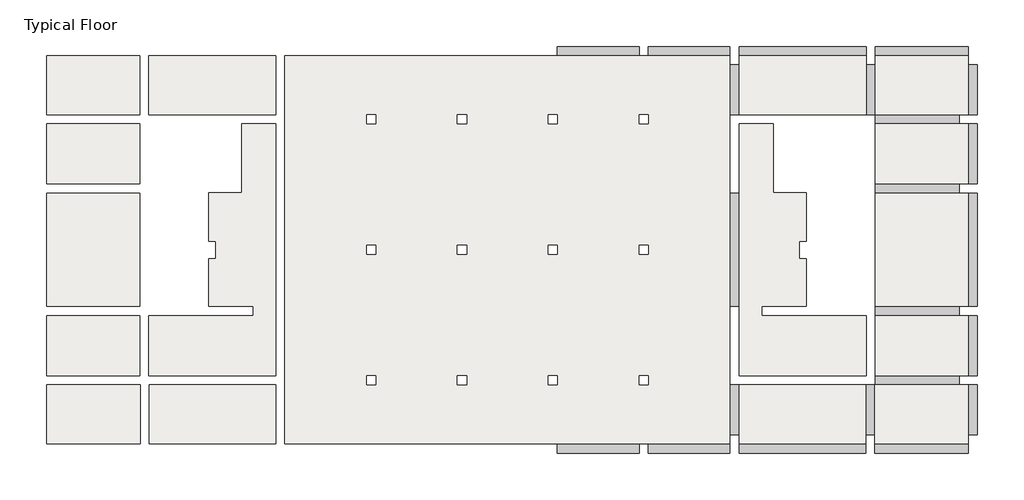
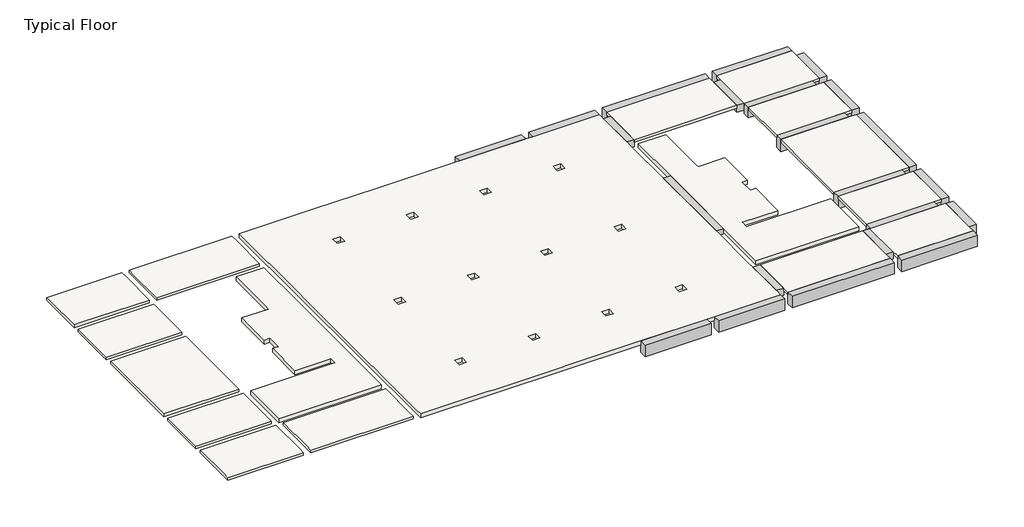
# One storey: 22 beams, 17 slabs.
"""IFC4 building model written with IfcOpenShell, lengths in millimetres."""

from ifc_helpers import new_model, si_unit, frame, origin, place, context, project, spatial, polyline, outline, extrude, faceted_brep, element, save

model = new_model("IFC4")

# Units and contexts
model_context = context("Model", 3, world=origin())
ifc_project = project(units=[si_unit("LENGTHUNIT", "METRE", prefix="MILLI")], contexts=[model_context])

# Site, building, storey
site = spatial("IfcSite", under=ifc_project)
building = spatial("IfcBuilding", under=site)
storey = spatial("IfcBuildingStorey", under=building, Name="Typical Floor", Elevation=4000.0)

# Beams
placement = place(None, origin())
element("IfcBeam", 1, ObjectType="Concrete Rectengular Beam : 40/30", at=placement, inside=storey, context=model_context, shape_type="SweptSolid", body=[
    extrude(outline(polyline([(9934.1113614, 5392.831899), (10334.1113614, 5392.831899), (10334.1113614, 443.9061014), (9934.1113614, 443.9061014), (9934.1113614, 5392.831899)])), frame((0.0, 0.0, 3700.0), z_axis=(0.0, 0.0, 1.0), x_axis=(1.0, 0.0, 0.0)), (0.0, 0.0, 1.0), 300.0),
])
element("IfcBeam", 2, ObjectType="Concrete Rectengular Beam : 40/40", at=placement, inside=storey, context=model_context, shape_type="Brep", body=[
    faceted_brep([(15855.0311968, -5152.7195656, 4000.0), (16255.0311968, -5152.7195656, 4000.0), (16255.0311968, -2974.5007845, 4000.0), (15855.0311968, -2974.5007845, 4000.0), (15855.0311968, -5152.7195656, 3600.0), (15855.0311968, -2974.5007845, 3600.0), (16255.0311968, -5152.7195656, 3600.0), (16255.0311968, -2974.5007845, 3600.0), (16255.0311968, -2974.5007845, 3850.0)], [[[0, 1, 2, 3]], [[4, 0, 3, 5]], [[6, 4, 5, 7]], [[1, 6, 7, 8, 2]], [[1, 0, 4, 6]], [[3, 2, 8, 7, 5]]]),
])
element("IfcBeam", 3, ObjectType="Concrete Rectengular Beam : 40/40", at=placement, inside=storey, context=model_context, shape_type="Brep", body=[
    faceted_brep([(9934.1113614, -5152.7195656, 4000.0), (10334.1113614, -5152.7195656, 4000.0), (10334.1113614, -2970.6647062, 4000.0), (9934.1113614, -2970.6647062, 4000.0), (9934.1113614, -5152.7195656, 3600.0), (9934.1113614, -2970.6647062, 3600.0), (10334.1113614, -5152.7195656, 3600.0), (10334.1113614, -2970.6647062, 3600.0), (10334.1113614, -2970.6647062, 3850.0)], [[[0, 1, 2, 3]], [[4, 0, 3, 5]], [[6, 4, 5, 7]], [[1, 6, 7, 8, 2]], [[1, 0, 4, 6]], [[3, 2, 8, 7, 5]]]),
])
element("IfcBeam", 4, ObjectType="Concrete Rectengular Beam : 40/40", at=placement, inside=storey, context=model_context, shape_type="Brep", body=[
    faceted_brep([(16276.5966375, 10981.7889465, 4000.0), (15876.5966375, 10981.7889465, 4000.0), (15876.5966375, 8813.6899891, 4000.0), (16276.5966375, 8813.6899891, 4000.0), (16276.5966375, 10981.7889465, 3600.0), (16276.5966375, 8813.6899891, 3850.0), (16276.5966375, 8813.6899891, 3600.0), (15876.5966375, 10981.7889465, 3600.0), (15876.5966375, 8813.6899891, 3600.0), (15876.5966375, 8813.6899891, 3850.0)], [[[0, 1, 2, 3]], [[4, 0, 3, 5, 6]], [[7, 4, 6, 8]], [[1, 7, 8, 9, 2]], [[1, 0, 4, 7]], [[3, 2, 9, 8, 6, 5]]]),
])
element("IfcBeam", 5, ObjectType="Concrete Rectengular Beam : 40/40", at=placement, inside=storey, context=model_context, shape_type="Brep", body=[
    faceted_brep([(10334.1113614, 10981.7889465, 4000.0), (9934.1113614, 10981.7889465, 4000.0), (9934.1113614, 8813.6899891, 4000.0), (10334.1113614, 8813.6899891, 4000.0), (10334.1113614, 10981.7889465, 3600.0), (10334.1113614, 8813.6899891, 3850.0), (10334.1113614, 8813.6899891, 3600.0), (9934.1113614, 10981.7889465, 3600.0), (9934.1113614, 8813.6899891, 3600.0)], [[[0, 1, 2, 3]], [[4, 0, 3, 5, 6]], [[7, 4, 6, 8]], [[1, 7, 8, 2]], [[1, 0, 4, 7]], [[3, 2, 8, 6, 5]]]),
])
element("IfcBeam", 6, ObjectType="Concrete Rectengular Beam : 40/60", at=placement, inside=storey, context=model_context, shape_type="Brep", body=[
    faceted_brep([(19935.0311968, 8413.6899891, 4000.0), (19935.0311968, 8813.6899891, 4000.0), (16276.5966375, 8813.6899891, 4000.0), (16276.5966375, 8413.6899891, 4000.0), (19935.0311968, 8413.6899891, 3400.0), (16276.5966375, 8413.6899891, 3850.0), (16276.5966375, 8413.6899891, 3400.0), (19935.0311968, 8813.6899891, 3400.0), (16276.5966375, 8813.6899891, 3400.0), (16276.5966375, 8813.6899891, 3850.0)], [[[0, 1, 2, 3]], [[4, 0, 3, 5, 6]], [[7, 4, 6, 8]], [[1, 7, 8, 9, 2]], [[1, 0, 4, 7]], [[3, 2, 9, 8, 6, 5]]]),
])
element("IfcBeam", 7, ObjectType="Concrete Rectengular Beam : 40/60", at=placement, inside=storey, context=model_context, shape_type="Brep", body=[
    faceted_brep([(19935.0311968, -2974.5007845, 4000.0), (19935.0311968, -2574.5007845, 4000.0), (16276.5966375, -2574.5007845, 4000.0), (16276.5966375, -2970.6647062, 4000.0), (15876.5966375, -2970.6647062, 4000.0), (15855.0311968, -2970.6647062, 4000.0), (15855.0311968, -2974.5007845, 4000.0), (16255.0311968, -2974.5007845, 4000.0), (19935.0311968, -2974.5007845, 3400.0), (15855.0311968, -2974.5007845, 3600.0), (15855.0311968, -2974.5007845, 3400.0), (19935.0311968, -2574.5007845, 3400.0), (15855.0311968, -2970.6647062, 3400.0), (16276.5966375, -2970.6647062, 3400.0), (16276.5966375, -2574.5007845, 3400.0), (15855.0311968, -2970.6647062, 3850.0), (16276.5966375, -2574.5007845, 3850.0)], [[[0, 1, 2, 3, 4, 5, 6, 7]], [[8, 0, 7, 6, 9, 10]], [[11, 8, 10, 12, 13, 14]], [[1, 0, 8, 11]], [[10, 9, 6, 5, 15, 12]], [[13, 3, 2, 16, 14]], [[3, 13, 12, 15, 5, 4]], [[1, 11, 14, 16, 2]]]),
])
element("IfcBeam", 8, ObjectType="Concrete Rectengular Beam : 40/65", at=placement, inside=storey, context=model_context, shape_type="Brep", body=[
    faceted_brep([(20335.0311968, 11381.7889465, 4000.0), (20335.0311968, 11781.7889465, 4000.0), (16276.5966375, 11781.7889465, 4000.0), (16276.5966375, 11381.7889465, 4000.0), (20335.0311968, 11781.7889465, 3350.0), (16276.5966375, 11781.7889465, 3350.0), (20335.0311968, 11381.7889465, 3350.0), (16276.5966375, 11381.7889465, 3350.0), (20335.0311968, 11381.7889465, 3850.0), (16276.5966375, 11381.7889465, 3850.0)], [[[0, 1, 2, 3]], [[1, 4, 5, 2]], [[4, 6, 7, 5]], [[6, 8, 0, 3, 9, 7]], [[1, 0, 8, 6, 4]], [[3, 2, 5, 7, 9]]]),
])
element("IfcBeam", 9, ObjectType="Concrete Rectengular Beam : 40/65", at=placement, inside=storey, context=model_context, shape_type="Brep", body=[
    faceted_brep([(15876.5966375, 11381.7889465, 4000.0), (15876.5966375, 11781.7889465, 4000.0), (10334.1113614, 11781.7889465, 4000.0), (10334.1113614, 11381.7889465, 4000.0), (15876.5966375, 11381.7889465, 3350.0), (15876.5966375, 11381.7889465, 3850.0), (10334.1113614, 11381.7889465, 3850.0), (10334.1113614, 11381.7889465, 3350.0), (15876.5966375, 11781.7889465, 3350.0), (10334.1113614, 11781.7889465, 3350.0)], [[[0, 1, 2, 3]], [[4, 5, 0, 3, 6, 7]], [[8, 4, 7, 9]], [[1, 8, 9, 2]], [[1, 0, 5, 4, 8]], [[3, 2, 9, 7, 6]]]),
])
element("IfcBeam", 10, ObjectType="Concrete Rectengular Beam : 40/65", at=placement, inside=storey, context=model_context, shape_type="Brep", body=[
    faceted_brep([(20335.0311968, -5948.8870638, 4000.0), (20335.0311968, -5548.8870638, 4000.0), (16255.0311968, -5548.8870638, 4000.0), (16255.0311968, -5948.8870638, 4000.0), (20335.0311968, -5948.8870638, 3350.0), (16255.0311968, -5948.8870638, 3350.0), (20335.0311968, -5548.8870638, 3350.0), (16255.0311968, -5548.8870638, 3350.0), (20335.0311968, -5548.8870638, 3850.0), (16255.0311968, -5548.8870638, 3850.0)], [[[0, 1, 2, 3]], [[4, 0, 3, 5]], [[6, 4, 5, 7]], [[1, 8, 6, 7, 9, 2]], [[1, 0, 4, 6, 8]], [[3, 2, 9, 7, 5]]]),
])
element("IfcBeam", 11, ObjectType="Concrete Rectengular Beam : 40/65", at=placement, inside=storey, context=model_context, shape_type="Brep", body=[
    faceted_brep([(15855.0311968, -5948.8870638, 4000.0), (15855.0311968, -5548.8870638, 4000.0), (10334.1113614, -5548.8870638, 4000.0), (10334.1113614, -5948.8870638, 4000.0), (15855.0311968, -5948.8870638, 3350.0), (10334.1113614, -5948.8870638, 3350.0), (15855.0311968, -5548.8870638, 3350.0), (10334.1113614, -5548.8870638, 3350.0), (15855.0311968, -5548.8870638, 3850.0), (10334.1113614, -5548.8870638, 3850.0)], [[[0, 1, 2, 3]], [[4, 0, 3, 5]], [[6, 4, 5, 7]], [[1, 8, 6, 7, 9, 2]], [[1, 0, 4, 6, 8]], [[3, 2, 9, 7, 5]]]),
])
element("IfcBeam", 12, ObjectType="Concrete Rectengular Beam : 40/65", at=placement, inside=storey, context=model_context, shape_type="Brep", body=[
    faceted_brep([(9934.1113614, 11381.7889465, 4000.0), (9934.1113614, 11781.7889465, 4000.0), (6372.4553623, 11781.7889465, 4000.0), (6372.4553623, 11381.7889465, 4000.0), (9934.1113614, 11381.7889465, 3350.0), (9934.1113614, 11381.7889465, 3770.0), (6372.4553623, 11381.7889465, 3350.0), (9934.1113614, 11781.7889465, 3350.0), (6372.4553623, 11781.7889465, 3350.0)], [[[0, 1, 2, 3]], [[4, 5, 0, 3, 6]], [[7, 4, 6, 8]], [[1, 7, 8, 2]], [[1, 0, 5, 4, 7]], [[3, 2, 8, 6]]]),
])
element("IfcBeam", 13, ObjectType="Concrete Rectengular Beam : 40/65", at=placement, inside=storey, context=model_context, shape_type="SweptSolid", body=[
    extrude(outline(polyline([(5972.4553623, 11781.7889465), (5972.4553623, 11381.7889465), (2410.7993238, 11381.7889465), (2410.7993238, 11781.7889465), (5972.4553623, 11781.7889465)])), frame((0.0, 0.0, 3350.0), z_axis=(0.0, 0.0, 1.0), x_axis=(1.0, 0.0, 0.0)), (0.0, 0.0, 1.0), 650.0),
])
element("IfcBeam", 14, ObjectType="Concrete Rectengular Beam : 40/65", at=placement, inside=storey, context=model_context, shape_type="Brep", body=[
    faceted_brep([(9934.1113614, -5948.8870638, 4000.0), (9934.1113614, -5548.8870638, 4000.0), (6372.4553623, -5548.8870638, 4000.0), (6372.4553623, -5948.8870638, 4000.0), (9934.1113614, -5948.8870638, 3350.0), (6372.4553623, -5948.8870638, 3350.0), (9934.1113614, -5548.8870638, 3350.0), (6372.4553623, -5548.8870638, 3350.0), (9934.1113614, -5548.8870638, 3770.0)], [[[0, 1, 2, 3]], [[4, 0, 3, 5]], [[6, 4, 5, 7]], [[1, 8, 6, 7, 2]], [[1, 0, 4, 6, 8]], [[3, 2, 7, 5]]]),
])
element("IfcBeam", 15, ObjectType="Concrete Rectengular Beam : 40/65", at=placement, inside=storey, context=model_context, shape_type="SweptSolid", body=[
    extrude(outline(polyline([(2410.7993238, -5948.8870638), (2410.7993238, -5548.8870638), (5972.4553623, -5548.8870638), (5972.4553623, -5948.8870638), (2410.7993238, -5948.8870638)])), frame((0.0, 0.0, 3350.0), z_axis=(0.0, 0.0, 1.0), x_axis=(1.0, 0.0, 0.0)), (0.0, 0.0, 1.0), 650.0),
])
element("IfcBeam", 16, ObjectType="Concrete Rectengular Beam : 40/65", at=placement, inside=storey, context=model_context, shape_type="Brep", body=[
    faceted_brep([(20735.0311968, 10981.7889465, 4000.0), (20335.0311968, 10981.7889465, 4000.0), (20335.0311968, 8813.6899891, 4000.0), (20735.0311968, 8813.6899891, 4000.0), (20735.0311968, 10981.7889465, 3350.0), (20735.0311968, 8813.6899891, 3350.0), (20335.0311968, 10981.7889465, 3350.0), (20335.0311968, 8813.6899891, 3350.0), (20335.0311968, 8813.6899891, 3850.0)], [[[0, 1, 2, 3]], [[4, 0, 3, 5]], [[6, 4, 5, 7]], [[1, 6, 7, 8, 2]], [[1, 0, 4, 6]], [[3, 2, 8, 7, 5]]]),
])
element("IfcBeam", 17, ObjectType="Concrete Rectengular Beam : 40/65", at=placement, inside=storey, context=model_context, shape_type="Brep", body=[
    faceted_brep([(20735.0311968, 8413.6899891, 4000.0), (20335.0311968, 8413.6899891, 4000.0), (20335.0311968, 5788.9969998, 4000.0), (20735.0311968, 5788.9969998, 4000.0), (20735.0311968, 8413.6899891, 3350.0), (20735.0311968, 5788.9969998, 3350.0), (20335.0311968, 8413.6899891, 3350.0), (20335.0311968, 5788.9969998, 3350.0), (20335.0311968, 8413.6899891, 3850.0), (20335.0311968, 5788.9969998, 3850.0)], [[[0, 1, 2, 3]], [[4, 0, 3, 5]], [[6, 4, 5, 7]], [[1, 8, 6, 7, 9, 2]], [[1, 0, 4, 6, 8]], [[3, 2, 9, 7, 5]]]),
])
element("IfcBeam", 18, ObjectType="Concrete Rectengular Beam : 40/65", at=placement, inside=storey, context=model_context, shape_type="Brep", body=[
    faceted_brep([(20735.0311968, 5388.9969998, 4000.0), (20335.0311968, 5388.9969998, 4000.0), (20335.0311968, 443.9061014, 4000.0), (20735.0311968, 443.9061014, 4000.0), (20735.0311968, 5388.9969998, 3350.0), (20735.0311968, 443.9061014, 3350.0), (20335.0311968, 5388.9969998, 3350.0), (20335.0311968, 443.9061014, 3350.0), (20335.0311968, 5388.9969998, 3850.0), (20335.0311968, 443.9061014, 3850.0)], [[[0, 1, 2, 3]], [[4, 0, 3, 5]], [[6, 4, 5, 7]], [[1, 8, 6, 7, 9, 2]], [[1, 0, 4, 6, 8]], [[3, 2, 9, 7, 5]]]),
])
element("IfcBeam", 19, ObjectType="Concrete Rectengular Beam : 40/65", at=placement, inside=storey, context=model_context, shape_type="Brep", body=[
    faceted_brep([(20735.0311968, 43.9061014, 4000.0), (20335.0311968, 43.9061014, 4000.0), (20335.0311968, -2574.5007845, 4000.0), (20735.0311968, -2574.5007845, 4000.0), (20735.0311968, 43.9061014, 3350.0), (20735.0311968, -2574.5007845, 3350.0), (20335.0311968, 43.9061014, 3350.0), (20335.0311968, -2574.5007845, 3350.0), (20335.0311968, 43.9061014, 3850.0), (20335.0311968, -2574.5007845, 3850.0)], [[[0, 1, 2, 3]], [[4, 0, 3, 5]], [[6, 4, 5, 7]], [[1, 8, 6, 7, 9, 2]], [[1, 0, 4, 6, 8]], [[3, 2, 9, 7, 5]]]),
])
element("IfcBeam", 20, ObjectType="Concrete Rectengular Beam : 40/65", at=placement, inside=storey, context=model_context, shape_type="Brep", body=[
    faceted_brep([(20735.0311968, -2974.5007845, 4000.0), (20335.0311968, -2974.5007845, 4000.0), (20335.0311968, -5152.7195656, 4000.0), (20735.0311968, -5152.7195656, 4000.0), (20735.0311968, -2974.5007845, 3350.0), (20735.0311968, -5152.7195656, 3350.0), (20335.0311968, -2974.5007845, 3350.0), (20335.0311968, -5152.7195656, 3350.0), (20335.0311968, -2974.5007845, 3850.0)], [[[0, 1, 2, 3]], [[4, 0, 3, 5]], [[6, 4, 5, 7]], [[1, 8, 6, 7, 2]], [[1, 0, 4, 6, 8]], [[3, 2, 7, 5]]]),
])
element("IfcBeam", 21, ObjectType="Concrete Rectengular Beam : 40/70", at=placement, inside=storey, context=model_context, shape_type="Brep", body=[
    faceted_brep([(19935.0311968, 43.9061014, 4000.0), (19935.0311968, 443.9061014, 4000.0), (16276.5966375, 443.9061014, 4000.0), (16276.5966375, 43.9061014, 4000.0), (19935.0311968, 43.9061014, 3300.0), (16276.5966375, 43.9061014, 3850.0), (16276.5966375, 43.9061014, 3300.0), (19935.0311968, 443.9061014, 3300.0), (16276.5966375, 443.9061014, 3300.0), (16276.5966375, 443.9061014, 3850.0)], [[[0, 1, 2, 3]], [[4, 0, 3, 5, 6]], [[7, 4, 6, 8]], [[1, 7, 8, 9, 2]], [[1, 0, 4, 7]], [[3, 2, 9, 8, 6, 5]]]),
])
element("IfcBeam", 22, ObjectType="Concrete Rectengular Beam : 40/70", at=placement, inside=storey, context=model_context, shape_type="Brep", body=[
    faceted_brep([(19935.0311968, 5388.9969998, 4000.0), (19935.0311968, 5788.9969998, 4000.0), (16276.5966375, 5788.9969998, 4000.0), (16276.5966375, 5388.9969998, 4000.0), (19935.0311968, 5388.9969998, 3300.0), (16276.5966375, 5388.9969998, 3850.0), (16276.5966375, 5388.9969998, 3300.0), (19935.0311968, 5788.9969998, 3300.0), (16276.5966375, 5788.9969998, 3300.0), (16276.5966375, 5788.9969998, 3850.0)], [[[0, 1, 2, 3]], [[4, 0, 3, 5, 6]], [[7, 4, 6, 8]], [[1, 7, 8, 9, 2]], [[1, 0, 4, 7]], [[3, 2, 9, 8, 6, 5]]]),
])

# Slabs
element("IfcSlab", 23, ObjectType="15", at=placement, inside=storey, context=model_context, shape_type="Brep", body=[
    faceted_brep([(-9870.3374688, 11381.7889465, 3850.0), (-9870.3374688, 8813.6899891, 3850.0), (-15412.8227448, 8813.6899891, 3850.0), (-15412.8227448, 11381.7889465, 3850.0), (-9870.3374688, 11381.7889465, 4000.0), (-15412.8227448, 11381.7889465, 4000.0), (-15412.8227448, 10981.7889465, 4000.0), (-15412.8227448, 8813.6899891, 4000.0), (-9870.3374688, 8813.6899891, 4000.0), (-9870.3374688, 10981.7889465, 4000.0)], [[[0, 1, 2, 3]], [[4, 5, 6, 7, 8, 9]], [[1, 0, 4, 9, 8]], [[2, 1, 8, 7]], [[3, 2, 7, 6, 5]], [[0, 3, 5, 4]]]),
])
element("IfcSlab", 24, ObjectType="15", at=placement, inside=storey, context=model_context, shape_type="Brep", body=[
    faceted_brep([(-15812.8227448, 11381.7889465, 3850.0), (-15812.8227448, 8813.6899891, 3850.0), (-19871.2573041, 8813.6899891, 3850.0), (-19871.2573041, 11381.7889465, 3850.0), (-15812.8227448, 11381.7889465, 4000.0), (-19871.2573041, 11381.7889465, 4000.0), (-19871.2573041, 10981.7889465, 4000.0), (-19871.2573041, 8813.6899891, 4000.0), (-19471.2573041, 8813.6899891, 4000.0), (-15812.8227448, 8813.6899891, 4000.0), (-15812.8227448, 10981.7889465, 4000.0)], [[[0, 1, 2, 3]], [[4, 5, 6, 7, 8, 9, 10]], [[1, 0, 4, 10, 9]], [[2, 1, 9, 8, 7]], [[3, 2, 7, 6, 5]], [[0, 3, 5, 4]]]),
])
element("IfcSlab", 25, ObjectType="15", at=placement, inside=storey, context=model_context, shape_type="Brep", body=[
    faceted_brep([(-15812.8227448, 8413.6899891, 3850.0), (-15812.8227448, 5788.9969998, 3850.0), (-19871.2573041, 5788.9969998, 3850.0), (-19871.2573041, 8413.6899891, 3850.0), (-15812.8227448, 8413.6899891, 4000.0), (-19471.2573041, 8413.6899891, 4000.0), (-19871.2573041, 8413.6899891, 4000.0), (-19871.2573041, 5788.9969998, 4000.0), (-19471.2573041, 5788.9969998, 4000.0), (-15812.8227448, 5788.9969998, 4000.0)], [[[0, 1, 2, 3]], [[4, 5, 6, 7, 8, 9]], [[1, 0, 4, 9]], [[2, 1, 9, 8, 7]], [[3, 2, 7, 6]], [[0, 3, 6, 5, 4]]]),
])
element("IfcSlab", 26, ObjectType="15", at=placement, inside=storey, context=model_context, shape_type="Brep", body=[
    faceted_brep([(-15812.8227448, 5388.9969998, 3850.0), (-15812.8227448, 443.9061014, 3850.0), (-19871.2573041, 443.9061014, 3850.0), (-19871.2573041, 5388.9969998, 3850.0), (-15812.8227448, 5388.9969998, 4000.0), (-19471.2573041, 5388.9969998, 4000.0), (-19871.2573041, 5388.9969998, 4000.0), (-19871.2573041, 443.9061014, 4000.0), (-19471.2573041, 443.9061014, 4000.0), (-15812.8227448, 443.9061014, 4000.0)], [[[0, 1, 2, 3]], [[4, 5, 6, 7, 8, 9]], [[1, 0, 4, 9]], [[2, 1, 9, 8, 7]], [[3, 2, 7, 6]], [[0, 3, 6, 5, 4]]]),
])
element("IfcSlab", 27, ObjectType="15", at=placement, inside=storey, context=model_context, shape_type="Brep", body=[
    faceted_brep([(-15791.2573041, -2974.5007845, 3850.0), (-15791.2573041, -5548.8870638, 3850.0), (-19871.2573041, -5548.8870638, 3850.0), (-19871.2573041, -2974.5007845, 3850.0), (-15791.2573041, -2974.5007845, 4000.0), (-19471.2573041, -2974.5007845, 4000.0), (-19871.2573041, -2974.5007845, 4000.0), (-19871.2573041, -5152.7195656, 4000.0), (-19871.2573041, -5548.8870638, 4000.0), (-15791.2573041, -5548.8870638, 4000.0), (-15791.2573041, -5152.7195656, 4000.0)], [[[0, 1, 2, 3]], [[4, 5, 6, 7, 8, 9, 10]], [[1, 0, 4, 10, 9]], [[2, 1, 9, 8]], [[3, 2, 8, 7, 6]], [[0, 3, 6, 5, 4]]]),
])
element("IfcSlab", 28, ObjectType="15", at=placement, inside=storey, context=model_context, shape_type="Brep", body=[
    faceted_brep([(-15812.8227448, 43.9061014, 3850.0), (-15812.8227448, -2574.5007845, 3850.0), (-19871.2573041, -2574.5007845, 3850.0), (-19871.2573041, 43.9061014, 3850.0), (-15812.8227448, 43.9061014, 4000.0), (-19471.2573041, 43.9061014, 4000.0), (-19871.2573041, 43.9061014, 4000.0), (-19871.2573041, -2574.5007845, 4000.0), (-19471.2573041, -2574.5007845, 4000.0), (-15812.8227448, -2574.5007845, 4000.0)], [[[0, 1, 2, 3]], [[4, 5, 6, 7, 8, 9]], [[1, 0, 4, 9]], [[2, 1, 9, 8, 7]], [[3, 2, 7, 6]], [[0, 3, 6, 5, 4]]]),
])
element("IfcSlab", 29, ObjectType="15", at=placement, inside=storey, context=model_context, shape_type="Brep", body=[
    faceted_brep([(-9870.3374688, -2970.6647062, 3850.0), (-9870.3374688, -5548.8870638, 3850.0), (-15391.2573041, -5548.8870638, 3850.0), (-15391.2573041, -2970.6647062, 3850.0), (-9870.3374688, -2970.6647062, 4000.0), (-15391.2573041, -2970.6647062, 4000.0), (-15391.2573041, -5152.7195656, 4000.0), (-15391.2573041, -5548.8870638, 4000.0), (-9870.3374688, -5548.8870638, 4000.0), (-9870.3374688, -5152.7195656, 4000.0)], [[[0, 1, 2, 3]], [[4, 5, 6, 7, 8, 9]], [[1, 0, 4, 9, 8]], [[2, 1, 8, 7]], [[3, 2, 7, 6, 5]], [[0, 3, 5, 4]]]),
])
element("IfcSlab", 30, ObjectType="15", at=placement, inside=storey, context=model_context, shape_type="Brep", body=[
    faceted_brep([(10334.1113614, 11381.7889465, 3850.0), (15876.5966375, 11381.7889465, 3850.0), (15876.5966375, 8813.6899891, 3850.0), (10334.1113614, 8813.6899891, 3850.0), (10334.1113614, 11381.7889465, 4000.0), (10334.1113614, 10981.7889465, 4000.0), (10334.1113614, 8813.6899891, 4000.0), (15876.5966375, 8813.6899891, 4000.0), (15876.5966375, 10981.7889465, 4000.0), (15876.5966375, 11381.7889465, 4000.0)], [[[0, 1, 2, 3]], [[4, 5, 6, 7, 8, 9]], [[0, 3, 6, 5, 4]], [[3, 2, 7, 6]], [[2, 1, 9, 8, 7]], [[1, 0, 4, 9]]]),
])
element("IfcSlab", 31, ObjectType="15", at=placement, inside=storey, context=model_context, shape_type="Brep", body=[
    faceted_brep([(16276.5966375, 11381.7889465, 3850.0), (20335.0311968, 11381.7889465, 3850.0), (20335.0311968, 8813.6899891, 3850.0), (16276.5966375, 8813.6899891, 3850.0), (16276.5966375, 11381.7889465, 4000.0), (16276.5966375, 10981.7889465, 4000.0), (16276.5966375, 8813.6899891, 4000.0), (19935.0311968, 8813.6899891, 4000.0), (20335.0311968, 8813.6899891, 4000.0), (20335.0311968, 10981.7889465, 4000.0), (20335.0311968, 11381.7889465, 4000.0)], [[[0, 1, 2, 3]], [[4, 5, 6, 7, 8, 9, 10]], [[0, 3, 6, 5, 4]], [[3, 2, 8, 7, 6]], [[2, 1, 10, 9, 8]], [[1, 0, 4, 10]]]),
])
element("IfcSlab", 32, ObjectType="15", at=placement, inside=storey, context=model_context, shape_type="Brep", body=[
    faceted_brep([(16276.5966375, 8413.6899891, 3850.0), (20335.0311968, 8413.6899891, 3850.0), (20335.0311968, 5788.9969998, 3850.0), (16276.5966375, 5788.9969998, 3850.0), (16276.5966375, 8413.6899891, 4000.0), (16276.5966375, 5788.9969998, 4000.0), (19935.0311968, 5788.9969998, 4000.0), (20335.0311968, 5788.9969998, 4000.0), (20335.0311968, 8413.6899891, 4000.0), (19935.0311968, 8413.6899891, 4000.0)], [[[0, 1, 2, 3]], [[4, 5, 6, 7, 8, 9]], [[0, 3, 5, 4]], [[3, 2, 7, 6, 5]], [[2, 1, 8, 7]], [[1, 0, 4, 9, 8]]]),
])
element("IfcSlab", 33, ObjectType="15", at=placement, inside=storey, context=model_context, shape_type="Brep", body=[
    faceted_brep([(16276.5966375, 5388.9969998, 3850.0), (20335.0311968, 5388.9969998, 3850.0), (20335.0311968, 443.9061014, 3850.0), (16276.5966375, 443.9061014, 3850.0), (16276.5966375, 5388.9969998, 4000.0), (16276.5966375, 443.9061014, 4000.0), (19935.0311968, 443.9061014, 4000.0), (20335.0311968, 443.9061014, 4000.0), (20335.0311968, 5388.9969998, 4000.0), (19935.0311968, 5388.9969998, 4000.0)], [[[0, 1, 2, 3]], [[4, 5, 6, 7, 8, 9]], [[0, 3, 5, 4]], [[3, 2, 7, 6, 5]], [[2, 1, 8, 7]], [[1, 0, 4, 9, 8]]]),
])
element("IfcSlab", 34, ObjectType="15", at=placement, inside=storey, context=model_context, shape_type="Brep", body=[
    faceted_brep([(16255.0311968, -2974.5007845, 3850.0), (20335.0311968, -2974.5007845, 3850.0), (20335.0311968, -5548.8870638, 3850.0), (16255.0311968, -5548.8870638, 3850.0), (16255.0311968, -2974.5007845, 4000.0), (16255.0311968, -5152.7195656, 4000.0), (16255.0311968, -5548.8870638, 4000.0), (20335.0311968, -5548.8870638, 4000.0), (20335.0311968, -5152.7195656, 4000.0), (20335.0311968, -2974.5007845, 4000.0), (19935.0311968, -2974.5007845, 4000.0)], [[[0, 1, 2, 3]], [[4, 5, 6, 7, 8, 9, 10]], [[0, 3, 6, 5, 4]], [[3, 2, 7, 6]], [[2, 1, 9, 8, 7]], [[1, 0, 4, 10, 9]]]),
])
element("IfcSlab", 35, ObjectType="15", at=placement, inside=storey, context=model_context, shape_type="Brep", body=[
    faceted_brep([(16276.5966375, 43.9061014, 3850.0), (20335.0311968, 43.9061014, 3850.0), (20335.0311968, -2574.5007845, 3850.0), (16276.5966375, -2574.5007845, 3850.0), (16276.5966375, 43.9061014, 4000.0), (16276.5966375, -2574.5007845, 4000.0), (19935.0311968, -2574.5007845, 4000.0), (20335.0311968, -2574.5007845, 4000.0), (20335.0311968, 43.9061014, 4000.0), (19935.0311968, 43.9061014, 4000.0)], [[[0, 1, 2, 3]], [[4, 5, 6, 7, 8, 9]], [[0, 3, 5, 4]], [[3, 2, 7, 6, 5]], [[2, 1, 8, 7]], [[1, 0, 4, 9, 8]]]),
])
element("IfcSlab", 36, ObjectType="15", at=placement, inside=storey, context=model_context, shape_type="Brep", body=[
    faceted_brep([(10334.1113614, -2970.6647062, 3850.0), (15855.0311968, -2970.6647062, 3850.0), (15855.0311968, -5548.8870638, 3850.0), (10334.1113614, -5548.8870638, 3850.0), (10334.1113614, -2970.6647062, 4000.0), (10334.1113614, -5152.7195656, 4000.0), (10334.1113614, -5548.8870638, 4000.0), (15855.0311968, -5548.8870638, 4000.0), (15855.0311968, -5152.7195656, 4000.0), (15855.0311968, -2974.5007845, 4000.0), (15855.0311968, -2970.6647062, 4000.0)], [[[0, 1, 2, 3]], [[4, 5, 6, 7, 8, 9, 10]], [[0, 3, 6, 5, 4]], [[3, 2, 7, 6]], [[2, 1, 10, 9, 8, 7]], [[1, 0, 4, 10]]]),
])
element("IfcSlab", 37, ObjectType="23", at=placement, inside=storey, context=model_context, shape_type="Brep", body=[
    faceted_brep([(9934.1113614, 11381.7889465, 3770.0), (9934.1113614, -5548.8870638, 3770.0), (-9470.3374688, -5548.8870638, 3770.0), (-9470.3374688, 11381.7889465, 3770.0), (-5508.6814696, 8413.6899891, 3770.0), (-5508.6814696, 8813.6899891, 3770.0), (-5908.6814696, 8813.6899891, 3770.0), (-5908.6814696, 8413.6899891, 3770.0), (-1547.0254312, 8413.6899891, 3770.0), (-1547.0254312, 8813.6899891, 3770.0), (-1947.0254312, 8813.6899891, 3770.0), (-1947.0254312, 8413.6899891, 3770.0), (-1547.0254312, 2716.4509414, 3770.0), (-1547.0254312, 3116.4509414, 3770.0), (-1947.0254312, 3116.4509414, 3770.0), (-1947.0254312, 2716.4509414, 3770.0), (-5508.6814696, 2716.4509414, 3770.0), (-5508.6814696, 3116.4509414, 3770.0), (-5908.6814696, 3116.4509414, 3770.0), (-5908.6814696, 2716.4509414, 3770.0), (-5508.6814696, -2974.5007845, 3770.0), (-5508.6814696, -2574.5007845, 3770.0), (-5908.6814696, -2574.5007845, 3770.0), (-5908.6814696, -2974.5007845, 3770.0), (-1547.0254312, -2974.5007845, 3770.0), (-1547.0254312, -2574.5007845, 3770.0), (-1947.0254312, -2574.5007845, 3770.0), (-1947.0254312, -2974.5007845, 3770.0), (5972.4553623, 8813.6899891, 3770.0), (5972.4553623, 8413.6899891, 3770.0), (6372.4553623, 8413.6899891, 3770.0), (6372.4553623, 8813.6899891, 3770.0), (2010.7993238, 8813.6899891, 3770.0), (2010.7993238, 8413.6899891, 3770.0), (2410.7993238, 8413.6899891, 3770.0), (2410.7993238, 8813.6899891, 3770.0), (2010.7993238, 3116.4509414, 3770.0), (2010.7993238, 2716.4509414, 3770.0), (2410.7993238, 2716.4509414, 3770.0), (2410.7993238, 3116.4509414, 3770.0), (5972.4553623, 3116.4509414, 3770.0), (5972.4553623, 2716.4509414, 3770.0), (6372.4553623, 2716.4509414, 3770.0), (6372.4553623, 3116.4509414, 3770.0), (5972.4553623, -2574.5007845, 3770.0), (5972.4553623, -2974.5007845, 3770.0), (6372.4553623, -2974.5007845, 3770.0), (6372.4553623, -2574.5007845, 3770.0), (2010.7993238, -2574.5007845, 3770.0), (2010.7993238, -2974.5007845, 3770.0), (2410.7993238, -2974.5007845, 3770.0), (2410.7993238, -2574.5007845, 3770.0), (9934.1113614, -5548.8870638, 4000.0), (9934.1113614, -5152.7195656, 4000.0), (9934.1113614, -2970.6647062, 4000.0), (9934.1113614, -2570.6647062, 4000.0), (9934.1113614, 443.9061014, 4000.0), (9934.1113614, 5392.831899, 4000.0), (9934.1113614, 8413.6899891, 4000.0), (9934.1113614, 8813.6899891, 4000.0), (9934.1113614, 10981.7889465, 4000.0), (9934.1113614, 11381.7889465, 4000.0), (6372.4553623, 11381.7889465, 4000.0), (5972.4553623, 11381.7889465, 4000.0), (2410.7993238, 11381.7889465, 4000.0), (2010.7993238, 11381.7889465, 4000.0), (-1547.0254312, 11381.7889465, 4000.0), (-1947.0254312, 11381.7889465, 4000.0), (-5508.6814696, 11381.7889465, 4000.0), (-5908.6814696, 11381.7889465, 4000.0), (-9470.3374688, 11381.7889465, 4000.0), (-9470.3374688, 10981.7889465, 4000.0), (-9470.3374688, 8813.6899891, 4000.0), (-9470.3374688, 8413.6899891, 4000.0), (-9470.3374688, 5392.831899, 4000.0), (-9470.3374688, 443.9061014, 4000.0), (-9470.3374688, -2570.6647062, 4000.0), (-9470.3374688, -2970.6647062, 4000.0), (-9470.3374688, -5152.7195656, 4000.0), (-9470.3374688, -5548.8870638, 4000.0), (-5908.6814696, -5548.8870638, 4000.0), (-5508.6814696, -5548.8870638, 4000.0), (-1947.0254312, -5548.8870638, 4000.0), (-1547.0254312, -5548.8870638, 4000.0), (2010.7993238, -5548.8870638, 4000.0), (2410.7993238, -5548.8870638, 4000.0), (5972.4553623, -5548.8870638, 4000.0), (6372.4553623, -5548.8870638, 4000.0), (-5508.6814696, 8813.6899891, 4000.0), (-5508.6814696, 8413.6899891, 4000.0), (-5908.6814696, 8413.6899891, 4000.0), (-5908.6814696, 8813.6899891, 4000.0), (-1547.0254312, 8813.6899891, 4000.0), (-1547.0254312, 8413.6899891, 4000.0), (-1947.0254312, 8413.6899891, 4000.0), (-1947.0254312, 8813.6899891, 4000.0), (-1547.0254312, 3116.4509414, 4000.0), (-1547.0254312, 2716.4509414, 4000.0), (-1947.0254312, 2716.4509414, 4000.0), (-1947.0254312, 3116.4509414, 4000.0), (-5508.6814696, 3116.4509414, 4000.0), (-5508.6814696, 2716.4509414, 4000.0), (-5908.6814696, 2716.4509414, 4000.0), (-5908.6814696, 3116.4509414, 4000.0), (-5508.6814696, -2574.5007845, 4000.0), (-5508.6814696, -2974.5007845, 4000.0), (-5908.6814696, -2974.5007845, 4000.0), (-5908.6814696, -2574.5007845, 4000.0), (-1547.0254312, -2574.5007845, 4000.0), (-1547.0254312, -2974.5007845, 4000.0), (-1947.0254312, -2974.5007845, 4000.0), (-1947.0254312, -2574.5007845, 4000.0), (5972.4553623, 8413.6899891, 4000.0), (5972.4553623, 8813.6899891, 4000.0), (6372.4553623, 8813.6899891, 4000.0), (6372.4553623, 8413.6899891, 4000.0), (2010.7993238, 8413.6899891, 4000.0), (2010.7993238, 8813.6899891, 4000.0), (2410.7993238, 8813.6899891, 4000.0), (2410.7993238, 8413.6899891, 4000.0), (2010.7993238, 2716.4509414, 4000.0), (2010.7993238, 3116.4509414, 4000.0), (2410.7993238, 3116.4509414, 4000.0), (2410.7993238, 2716.4509414, 4000.0), (5972.4553623, 2716.4509414, 4000.0), (5972.4553623, 3116.4509414, 4000.0), (6372.4553623, 3116.4509414, 4000.0), (6372.4553623, 2716.4509414, 4000.0), (5972.4553623, -2974.5007845, 4000.0), (5972.4553623, -2574.5007845, 4000.0), (6372.4553623, -2574.5007845, 4000.0), (6372.4553623, -2974.5007845, 4000.0), (2010.7993238, -2974.5007845, 4000.0), (2010.7993238, -2574.5007845, 4000.0), (2410.7993238, -2574.5007845, 4000.0), (2410.7993238, -2974.5007845, 4000.0)], [[[0, 1, 2, 3], [4, 5, 6, 7], [8, 9, 10, 11], [12, 13, 14, 15], [16, 17, 18, 19], [20, 21, 22, 23], [24, 25, 26, 27], [28, 29, 30, 31], [32, 33, 34, 35], [36, 37, 38, 39], [40, 41, 42, 43], [44, 45, 46, 47], [48, 49, 50, 51]], [[52, 53, 54, 55, 56, 57, 58, 59, 60, 61, 62, 63, 64, 65, 66, 67, 68, 69, 70, 71, 72, 73, 74, 75, 76, 77, 78, 79, 80, 81, 82, 83, 84, 85, 86, 87], [88, 89, 90, 91], [92, 93, 94, 95], [96, 97, 98, 99], [100, 101, 102, 103], [104, 105, 106, 107], [108, 109, 110, 111], [112, 113, 114, 115], [116, 117, 118, 119], [120, 121, 122, 123], [124, 125, 126, 127], [128, 129, 130, 131], [132, 133, 134, 135]], [[1, 0, 61, 60, 59, 58, 57, 56, 55, 54, 53, 52]], [[2, 1, 52, 87, 86, 85, 84, 83, 82, 81, 80, 79]], [[3, 2, 79, 78, 77, 76, 75, 74, 73, 72, 71, 70]], [[0, 3, 70, 69, 68, 67, 66, 65, 64, 63, 62, 61]], [[4, 89, 88, 5]], [[89, 4, 7, 90]], [[90, 7, 6, 91]], [[91, 6, 5, 88]], [[8, 93, 92, 9]], [[93, 8, 11, 94]], [[94, 11, 10, 95]], [[95, 10, 9, 92]], [[12, 97, 96, 13]], [[97, 12, 15, 98]], [[98, 15, 14, 99]], [[99, 14, 13, 96]], [[16, 101, 100, 17]], [[101, 16, 19, 102]], [[102, 19, 18, 103]], [[103, 18, 17, 100]], [[20, 105, 104, 21]], [[105, 20, 23, 106]], [[106, 23, 22, 107]], [[107, 22, 21, 104]], [[24, 109, 108, 25]], [[109, 24, 27, 110]], [[110, 27, 26, 111]], [[111, 26, 25, 108]], [[112, 29, 28, 113]], [[29, 112, 115, 30]], [[30, 115, 114, 31]], [[31, 114, 113, 28]], [[116, 33, 32, 117]], [[33, 116, 119, 34]], [[34, 119, 118, 35]], [[35, 118, 117, 32]], [[120, 37, 36, 121]], [[37, 120, 123, 38]], [[38, 123, 122, 39]], [[39, 122, 121, 36]], [[124, 41, 40, 125]], [[41, 124, 127, 42]], [[42, 127, 126, 43]], [[43, 126, 125, 40]], [[128, 45, 44, 129]], [[45, 128, 131, 46]], [[46, 131, 130, 47]], [[47, 130, 129, 44]], [[132, 49, 48, 133]], [[49, 132, 135, 50]], [[50, 135, 134, 51]], [[51, 134, 133, 48]]]),
])
element("IfcSlab", 38, ObjectType="23", at=placement, inside=storey, context=model_context, shape_type="Brep", body=[
    faceted_brep([(-11354.3869672, 8413.6899891, 3770.0), (-9870.3374688, 8413.6899891, 3770.0), (-9870.3374688, -2570.6647062, 3770.0), (-15412.8227448, -2570.6647062, 3770.0), (-15412.8227448, 43.9061014, 3770.0), (-10863.8957288, 43.9061014, 3770.0), (-10863.8957288, 443.9061014, 3770.0), (-12794.417038, 443.9061014, 3770.0), (-12794.417038, 2525.3463223, 3770.0), (-12498.865318, 2525.3463223, 3770.0), (-12498.865318, 3298.8134973, 3770.0), (-12794.417038, 3298.8134973, 3770.0), (-12794.417038, 5394.6720806, 3770.0), (-11354.3869672, 5394.6720806, 3770.0), (-11354.3869672, 5694.6720806, 3770.0), (-9870.3374688, 8413.6899891, 4000.0), (-11354.3869672, 8413.6899891, 4000.0), (-11354.3869672, 5694.6720806, 4000.0), (-11354.3869672, 5394.6720806, 4000.0), (-12794.417038, 5394.6720806, 4000.0), (-12794.417038, 3298.8134973, 4000.0), (-12498.865318, 3298.8134973, 4000.0), (-12498.865318, 2525.3463223, 4000.0), (-12794.417038, 2525.3463223, 4000.0), (-12794.417038, 443.9061014, 4000.0), (-10863.8957288, 443.9061014, 4000.0), (-10863.8957288, 43.9061014, 4000.0), (-15412.8227448, 43.9061014, 4000.0), (-15412.8227448, -2570.6647062, 4000.0), (-9870.3374688, -2570.6647062, 4000.0), (-9870.3374688, 443.9061014, 4000.0), (-9870.3374688, 5392.831899, 4000.0)], [[[0, 1, 2, 3, 4, 5, 6, 7, 8, 9, 10, 11, 12, 13, 14]], [[15, 16, 17, 18, 19, 20, 21, 22, 23, 24, 25, 26, 27, 28, 29, 30, 31]], [[1, 0, 16, 15]], [[1, 15, 31, 30, 29, 2]], [[25, 6, 5, 26]], [[7, 6, 25, 24]], [[7, 24, 23, 8]], [[19, 12, 11, 20]], [[13, 12, 19, 18]], [[13, 18, 17, 16, 0, 14]], [[3, 28, 27, 4]], [[3, 2, 29, 28]], [[26, 5, 4, 27]], [[9, 22, 21, 10]], [[22, 9, 8, 23]], [[10, 21, 20, 11]]]),
])
element("IfcSlab", 39, ObjectType="23", at=placement, inside=storey, context=model_context, shape_type="Brep", body=[
    faceted_brep([(10334.1113614, 8413.6899891, 3770.0), (11818.1608598, 8413.6899891, 3770.0), (11818.1608598, 5694.6720806, 3770.0), (11818.1608598, 5394.6720806, 3770.0), (13258.1909307, 5394.6720806, 3770.0), (13258.1909307, 3298.8134973, 3770.0), (12962.6392106, 3298.8134973, 3770.0), (12962.6392106, 2525.3463223, 3770.0), (13258.1909307, 2525.3463223, 3770.0), (13258.1909307, 443.9061014, 3770.0), (11327.6696215, 443.9061014, 3770.0), (11327.6696215, 43.9061014, 3770.0), (15876.5966375, 43.9061014, 3770.0), (15876.5966375, -2570.6647062, 3770.0), (10334.1113614, -2570.6647062, 3770.0), (11818.1608598, 8413.6899891, 4000.0), (10334.1113614, 8413.6899891, 4000.0), (10334.1113614, 5392.831899, 4000.0), (10334.1113614, 443.9061014, 4000.0), (10334.1113614, -2570.6647062, 4000.0), (15876.5966375, -2570.6647062, 4000.0), (15876.5966375, 43.9061014, 4000.0), (11327.6696215, 43.9061014, 4000.0), (11327.6696215, 443.9061014, 4000.0), (13258.1909307, 443.9061014, 4000.0), (13258.1909307, 2525.3463223, 4000.0), (12962.6392106, 2525.3463223, 4000.0), (12962.6392106, 3298.8134973, 4000.0), (13258.1909307, 3298.8134973, 4000.0), (13258.1909307, 5394.6720806, 4000.0), (11818.1608598, 5394.6720806, 4000.0), (11818.1608598, 5694.6720806, 4000.0)], [[[0, 1, 2, 3, 4, 5, 6, 7, 8, 9, 10, 11, 12, 13, 14]], [[15, 16, 17, 18, 19, 20, 21, 22, 23, 24, 25, 26, 27, 28, 29, 30, 31]], [[1, 0, 16, 15]], [[16, 0, 14, 19, 18, 17]], [[10, 23, 22, 11]], [[10, 9, 24, 23]], [[4, 29, 28, 5]], [[24, 9, 8, 25]], [[4, 3, 30, 29]], [[30, 3, 2, 1, 15, 31]], [[20, 13, 12, 21]], [[14, 13, 20, 19]], [[11, 22, 21, 12]], [[6, 27, 26, 7]], [[7, 26, 25, 8]], [[27, 6, 5, 28]]]),
])

save(model, "model.ifc")

# Revit data of these elements
# Type "Concrete Rectengular Beam : 40/30"
#   Length [instance default] = 152.4 cm
#   b = 40 cm
#   h = 30 cm
#   Structural Material [instance default] = Concrete
#   Assembly Code = ""
# Type "Concrete Rectengular Beam : 40/40"
#   Length [instance default] = 152.4 cm
#   b = 40 cm
#   h = 40 cm
#   Structural Material [instance default] = Concrete
#   Assembly Code = ""
# Type "Concrete Rectengular Beam : 40/60"
#   Length [instance default] = 152.4 cm
#   b = 40 cm
#   h = 60 cm
#   Structural Material [instance default] = Concrete
#   Assembly Code = ""
# Type "Concrete Rectengular Beam : 40/65"
#   Length [instance default] = 152.4 cm
#   b = 40 cm
#   h = 65 cm
#   Structural Material [instance default] = Concrete
#   Assembly Code = ""
# Type "Concrete Rectengular Beam : 40/70"
#   Length [instance default] = 152.4 cm
#   b = 40 cm
#   h = 70 cm
#   Structural Material [instance default] = Concrete
#   Assembly Code = ""
# Type "15"
#   Function = 0
#   Layers, outside or top first: 15 cm "Concrete" (function 1)
# Type "23"
#   Function = 0
#   Layers, outside or top first: 23 cm "Concrete" (function 1)
# Element 1 (IfcBeam, "Concrete Rectengular Beam : 40/30")
#   Comments = ""
#   Mark = "B2"
#   SOFiSTiK_AMG_Comments = ""
#   SOFiSTiK_AMG_Scheduled = yes
#   SOFiSTiK_AMG_Adjusted = yes
#   Structural Material = Concrete
#   Phase Created = New Construction
#   Materials on its faces: "Concrete"
# Element 2 (IfcBeam, "Concrete Rectengular Beam : 40/40")
#   Comments = ""
#   Mark = "B7"
#   SOFiSTiK_AMG_Comments = ""
#   SOFiSTiK_AMG_Scheduled = yes
#   SOFiSTiK_AMG_Adjusted = yes
#   Structural Material = Concrete
#   Phase Created = New Construction
#   Materials on its faces: "Concrete"
# Element 3 (IfcBeam, "Concrete Rectengular Beam : 40/40")
#   Comments = ""
#   Mark = "B8"
#   SOFiSTiK_AMG_Comments = ""
#   SOFiSTiK_AMG_Scheduled = yes
#   SOFiSTiK_AMG_Adjusted = yes
#   Structural Material = Concrete
#   Phase Created = New Construction
#   Materials on its faces: "Concrete"
# Element 4 (IfcBeam, "Concrete Rectengular Beam : 40/40")
#   Comments = ""
#   Mark = "B9"
#   SOFiSTiK_AMG_Comments = ""
#   SOFiSTiK_AMG_Scheduled = yes
#   SOFiSTiK_AMG_Adjusted = yes
#   Structural Material = Concrete
#   Phase Created = New Construction
#   Materials on its faces: "Concrete"
# Element 5 (IfcBeam, "Concrete Rectengular Beam : 40/40")
#   Comments = ""
#   Mark = "B10"
#   SOFiSTiK_AMG_Comments = ""
#   SOFiSTiK_AMG_Scheduled = yes
#   SOFiSTiK_AMG_Adjusted = yes
#   Structural Material = Concrete
#   Phase Created = New Construction
#   Materials on its faces: "Concrete"
# Element 6 (IfcBeam, "Concrete Rectengular Beam : 40/60")
#   Comments = ""
#   Mark = "B13"
#   SOFiSTiK_AMG_Comments = ""
#   SOFiSTiK_AMG_Scheduled = yes
#   SOFiSTiK_AMG_Adjusted = yes
#   Structural Material = Concrete
#   Phase Created = New Construction
#   Materials on its faces: "Concrete"
# Element 7 (IfcBeam, "Concrete Rectengular Beam : 40/60")
#   Comments = ""
#   Mark = "B14"
#   SOFiSTiK_AMG_Comments = ""
#   SOFiSTiK_AMG_Scheduled = yes
#   SOFiSTiK_AMG_Adjusted = yes
#   Structural Material = Concrete
#   Phase Created = New Construction
#   Materials on its faces: "Concrete"
# Element 8 (IfcBeam, "Concrete Rectengular Beam : 40/65")
#   Comments = ""
#   Mark = "B28"
#   SOFiSTiK_AMG_Comments = ""
#   SOFiSTiK_AMG_Scheduled = yes
#   SOFiSTiK_AMG_Adjusted = yes
#   Structural Material = Concrete
#   Phase Created = New Construction
#   Materials on its faces: "Concrete"
# Element 9 (IfcBeam, "Concrete Rectengular Beam : 40/65")
#   Comments = ""
#   Mark = "B29"
#   SOFiSTiK_AMG_Comments = ""
#   SOFiSTiK_AMG_Scheduled = yes
#   SOFiSTiK_AMG_Adjusted = yes
#   Structural Material = Concrete
#   Phase Created = New Construction
#   Materials on its faces: "Concrete"
# Element 10 (IfcBeam, "Concrete Rectengular Beam : 40/65")
#   Comments = ""
#   Mark = "B30"
#   SOFiSTiK_AMG_Comments = ""
#   SOFiSTiK_AMG_Scheduled = yes
#   SOFiSTiK_AMG_Adjusted = yes
#   Structural Material = Concrete
#   Phase Created = New Construction
#   Materials on its faces: "Concrete"
# Element 11 (IfcBeam, "Concrete Rectengular Beam : 40/65")
#   Comments = ""
#   Mark = "B31"
#   SOFiSTiK_AMG_Comments = ""
#   SOFiSTiK_AMG_Scheduled = yes
#   SOFiSTiK_AMG_Adjusted = yes
#   Structural Material = Concrete
#   Phase Created = New Construction
#   Materials on its faces: "Concrete"
# Element 12 (IfcBeam, "Concrete Rectengular Beam : 40/65")
#   Comments = ""
#   Mark = "B32"
#   SOFiSTiK_AMG_Comments = ""
#   SOFiSTiK_AMG_Scheduled = yes
#   SOFiSTiK_AMG_Adjusted = yes
#   Structural Material = Concrete
#   Phase Created = New Construction
#   Materials on its faces: "Concrete"
# Element 13 (IfcBeam, "Concrete Rectengular Beam : 40/65")
#   Comments = ""
#   Mark = "B33"
#   SOFiSTiK_AMG_Comments = ""
#   SOFiSTiK_AMG_Scheduled = yes
#   SOFiSTiK_AMG_Adjusted = yes
#   Structural Material = Concrete
#   Phase Created = New Construction
#   Materials on its faces: "Concrete"
# Element 14 (IfcBeam, "Concrete Rectengular Beam : 40/65")
#   Comments = ""
#   Mark = "B34"
#   SOFiSTiK_AMG_Comments = ""
#   SOFiSTiK_AMG_Scheduled = yes
#   SOFiSTiK_AMG_Adjusted = yes
#   Structural Material = Concrete
#   Phase Created = New Construction
#   Materials on its faces: "Concrete"
# Element 15 (IfcBeam, "Concrete Rectengular Beam : 40/65")
#   Comments = ""
#   Mark = "B35"
#   SOFiSTiK_AMG_Comments = ""
#   SOFiSTiK_AMG_Scheduled = yes
#   SOFiSTiK_AMG_Adjusted = yes
#   Structural Material = Concrete
#   Phase Created = New Construction
#   Materials on its faces: "Concrete"
# Element 16 (IfcBeam, "Concrete Rectengular Beam : 40/65")
#   Comments = ""
#   Mark = "B36"
#   SOFiSTiK_AMG_Comments = ""
#   SOFiSTiK_AMG_Scheduled = yes
#   SOFiSTiK_AMG_Adjusted = yes
#   Structural Material = Concrete
#   Phase Created = New Construction
#   Materials on its faces: "Concrete"
# Element 17 (IfcBeam, "Concrete Rectengular Beam : 40/65")
#   Comments = ""
#   Mark = "B37"
#   SOFiSTiK_AMG_Comments = ""
#   SOFiSTiK_AMG_Scheduled = yes
#   SOFiSTiK_AMG_Adjusted = yes
#   Structural Material = Concrete
#   Phase Created = New Construction
#   Materials on its faces: "Concrete"
# Element 18 (IfcBeam, "Concrete Rectengular Beam : 40/65")
#   Comments = ""
#   Mark = "B38"
#   SOFiSTiK_AMG_Comments = ""
#   SOFiSTiK_AMG_Scheduled = yes
#   SOFiSTiK_AMG_Adjusted = yes
#   Structural Material = Concrete
#   Phase Created = New Construction
#   Materials on its faces: "Concrete"
# Element 19 (IfcBeam, "Concrete Rectengular Beam : 40/65")
#   Comments = ""
#   Mark = "B39"
#   SOFiSTiK_AMG_Comments = ""
#   SOFiSTiK_AMG_Scheduled = yes
#   SOFiSTiK_AMG_Adjusted = yes
#   Structural Material = Concrete
#   Phase Created = New Construction
#   Materials on its faces: "Concrete"
# Element 20 (IfcBeam, "Concrete Rectengular Beam : 40/65")
#   Comments = ""
#   Mark = "B40"
#   SOFiSTiK_AMG_Comments = ""
#   SOFiSTiK_AMG_Scheduled = yes
#   SOFiSTiK_AMG_Adjusted = yes
#   Structural Material = Concrete
#   Phase Created = New Construction
#   Materials on its faces: "Concrete"
# Element 21 (IfcBeam, "Concrete Rectengular Beam : 40/70")
#   Comments = ""
#   Mark = "B45"
#   SOFiSTiK_AMG_Comments = ""
#   SOFiSTiK_AMG_Scheduled = yes
#   SOFiSTiK_AMG_Adjusted = yes
#   Structural Material = Concrete
#   Phase Created = New Construction
#   Materials on its faces: "Concrete"
# Element 22 (IfcBeam, "Concrete Rectengular Beam : 40/70")
#   Comments = ""
#   Mark = "B46"
#   SOFiSTiK_AMG_Comments = ""
#   SOFiSTiK_AMG_Scheduled = yes
#   SOFiSTiK_AMG_Adjusted = yes
#   Structural Material = Concrete
#   Phase Created = New Construction
#   Materials on its faces: "Concrete"
# Element 23 (IfcSlab, "15")
#   Mark = "S1"
#   SOFiSTiK_AMG_Comments = ""
#   Height Offset From Level = 0 cm
#   built-in parameter 1001954 = 1
#   SOFiSTiK_AMG_Scheduled = yes
#   SOFiSTiK_AMG_Adjusted = yes
#   Phase Created = New Construction
#   Materials on its faces: "Concrete"
# Element 24 (IfcSlab, "15")
#   Mark = "S2"
#   SOFiSTiK_AMG_Comments = ""
#   Height Offset From Level = 0 cm
#   built-in parameter 1001954 = 1
#   SOFiSTiK_AMG_Scheduled = yes
#   SOFiSTiK_AMG_Adjusted = yes
#   Phase Created = New Construction
#   Materials on its faces: "Concrete"
# Element 25 (IfcSlab, "15")
#   Mark = "S3"
#   SOFiSTiK_AMG_Comments = ""
#   Height Offset From Level = 0 cm
#   built-in parameter 1001954 = 1
#   SOFiSTiK_AMG_Scheduled = yes
#   SOFiSTiK_AMG_Adjusted = yes
#   Phase Created = New Construction
#   Materials on its faces: "Concrete"
# Element 26 (IfcSlab, "15")
#   Mark = "S4"
#   SOFiSTiK_AMG_Comments = ""
#   Height Offset From Level = 0 cm
#   built-in parameter 1001954 = 1
#   SOFiSTiK_AMG_Scheduled = yes
#   SOFiSTiK_AMG_Adjusted = yes
#   Phase Created = New Construction
#   Materials on its faces: "Concrete"
# Element 27 (IfcSlab, "15")
#   Mark = "S5"
#   SOFiSTiK_AMG_Comments = ""
#   Height Offset From Level = 0 cm
#   built-in parameter 1001954 = 1
#   SOFiSTiK_AMG_Scheduled = yes
#   SOFiSTiK_AMG_Adjusted = yes
#   Phase Created = New Construction
#   Materials on its faces: "Concrete"
# Element 28 (IfcSlab, "15")
#   Mark = "S6"
#   SOFiSTiK_AMG_Comments = ""
#   Height Offset From Level = 0 cm
#   built-in parameter 1001954 = 1
#   SOFiSTiK_AMG_Scheduled = yes
#   SOFiSTiK_AMG_Adjusted = yes
#   Phase Created = New Construction
#   Materials on its faces: "Concrete"
# Element 29 (IfcSlab, "15")
#   Mark = "S7"
#   SOFiSTiK_AMG_Comments = ""
#   Height Offset From Level = 0 cm
#   built-in parameter 1001954 = 1
#   SOFiSTiK_AMG_Scheduled = yes
#   SOFiSTiK_AMG_Adjusted = yes
#   Phase Created = New Construction
#   Materials on its faces: "Concrete"
# Element 30 (IfcSlab, "15")
#   Mark = "S8"
#   SOFiSTiK_AMG_Comments = ""
#   built-in parameter 1001955 = 3.14159 (stored number, unit not read)
#   Height Offset From Level = 0 cm
#   built-in parameter 1001954 = 1
#   SOFiSTiK_AMG_Scheduled = yes
#   SOFiSTiK_AMG_Adjusted = yes
#   Phase Created = New Construction
#   Materials on its faces: "Concrete"
# Element 31 (IfcSlab, "15")
#   Mark = "S9"
#   SOFiSTiK_AMG_Comments = ""
#   built-in parameter 1001955 = 3.14159 (stored number, unit not read)
#   Height Offset From Level = 0 cm
#   built-in parameter 1001954 = 1
#   SOFiSTiK_AMG_Scheduled = yes
#   SOFiSTiK_AMG_Adjusted = yes
#   Phase Created = New Construction
#   Materials on its faces: "Concrete"
# Element 32 (IfcSlab, "15")
#   Mark = "S10"
#   SOFiSTiK_AMG_Comments = ""
#   built-in parameter 1001955 = 3.14159 (stored number, unit not read)
#   Height Offset From Level = 0 cm
#   built-in parameter 1001954 = 1
#   SOFiSTiK_AMG_Scheduled = yes
#   SOFiSTiK_AMG_Adjusted = yes
#   Phase Created = New Construction
#   Materials on its faces: "Concrete"
# Element 33 (IfcSlab, "15")
#   Mark = "S11"
#   SOFiSTiK_AMG_Comments = ""
#   built-in parameter 1001955 = 3.14159 (stored number, unit not read)
#   Height Offset From Level = 0 cm
#   built-in parameter 1001954 = 1
#   SOFiSTiK_AMG_Scheduled = yes
#   SOFiSTiK_AMG_Adjusted = yes
#   Phase Created = New Construction
#   Materials on its faces: "Concrete"
# Element 34 (IfcSlab, "15")
#   Mark = "S12"
#   SOFiSTiK_AMG_Comments = ""
#   built-in parameter 1001955 = 3.14159 (stored number, unit not read)
#   Height Offset From Level = 0 cm
#   built-in parameter 1001954 = 1
#   SOFiSTiK_AMG_Scheduled = yes
#   SOFiSTiK_AMG_Adjusted = yes
#   Phase Created = New Construction
#   Materials on its faces: "Concrete"
# Element 35 (IfcSlab, "15")
#   Mark = "S13"
#   SOFiSTiK_AMG_Comments = ""
#   built-in parameter 1001955 = 3.14159 (stored number, unit not read)
#   Height Offset From Level = 0 cm
#   built-in parameter 1001954 = 1
#   SOFiSTiK_AMG_Scheduled = yes
#   SOFiSTiK_AMG_Adjusted = yes
#   Phase Created = New Construction
#   Materials on its faces: "Concrete"
# Element 36 (IfcSlab, "15")
#   Mark = "S14"
#   SOFiSTiK_AMG_Comments = ""
#   built-in parameter 1001955 = 3.14159 (stored number, unit not read)
#   Height Offset From Level = 0 cm
#   built-in parameter 1001954 = 1
#   SOFiSTiK_AMG_Scheduled = yes
#   SOFiSTiK_AMG_Adjusted = yes
#   Phase Created = New Construction
#   Materials on its faces: "Concrete"
# Element 37 (IfcSlab, "23")
#   Mark = "S15"
#   SOFiSTiK_AMG_Comments = ""
#   Height Offset From Level = 0 cm
#   built-in parameter 1001954 = 1
#   SOFiSTiK_AMG_Scheduled = yes
#   SOFiSTiK_AMG_Adjusted = yes
#   Phase Created = New Construction
#   Materials on its faces: "Concrete"
# Element 38 (IfcSlab, "23")
#   Mark = "S16"
#   SOFiSTiK_AMG_Comments = ""
#   built-in parameter 1001955 = 3.14159 (stored number, unit not read)
#   Height Offset From Level = 0 cm
#   built-in parameter 1001954 = 1
#   SOFiSTiK_AMG_Scheduled = yes
#   SOFiSTiK_AMG_Adjusted = yes
#   Phase Created = New Construction
#   Materials on its faces: "Concrete"
# Element 39 (IfcSlab, "23")
#   Mark = "S17"
#   SOFiSTiK_AMG_Comments = ""
#   built-in parameter 1001955 = 0 (stored number, unit not read)
#   Height Offset From Level = 0 cm
#   built-in parameter 1001954 = 1
#   SOFiSTiK_AMG_Scheduled = yes
#   SOFiSTiK_AMG_Adjusted = yes
#   Phase Created = New Construction
#   Materials on its faces: "Concrete"
# Materials
#   "Concrete": class "Concrete", colour RGB 192 192 192, transparency 0, Keynote = "01000", Description = "Cast-in-place concrete", Cost = 0
